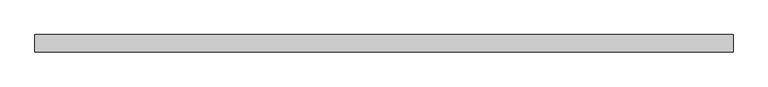
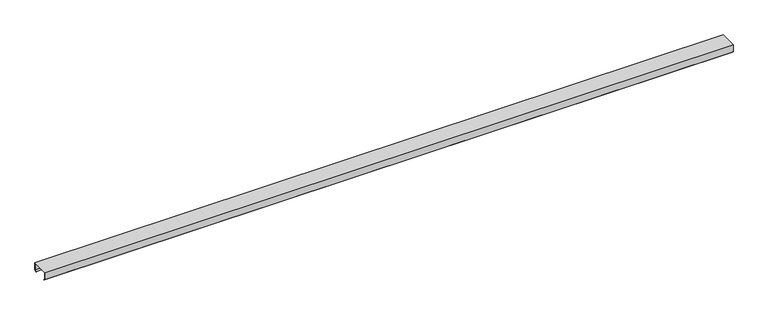
"""IFC4 building model written with IfcOpenShell, lengths in millimetres: proxy geometry, Generic Models 7:Generic Models 1:1:Generic Models 1:1 : Generic Models 7:Generic Models 1:337419:38 : Generic Models 7:Generic Models 1:1:Generic Models 1:1 : Generic Models 7:Generic Models 1:337419:306201."""

from ifc_helpers import new_model, si_unit, frame, origin, place, context, project, spatial, polyline, outline, extrude, source, transform, mapped, element, save


def generic_models_92c28086(model_context):
    return source(origin(), model_context, "Body", "SweptSolid", [
        extrude(outline(polyline([(-578797.4913841, 4985.940625), (-578797.4913841, 4897.040625), (-578812.0845307, 4884.7955211), (-578813.870275, 4886.9236883), (-578800.2695091, 4898.336086), (-578800.2695091, 4983.1625), (-578997.9132591, 4983.1625), (-578997.9132591, 4898.336086), (-578984.3124931, 4886.9236883), (-578986.0982374, 4884.7955211), (-579000.6913841, 4897.040625), (-579000.6913841, 4985.940625), (-578797.4913841, 4985.940625)])), frame((795954.8382438, 0.0, 0.0), z_axis=(1.0, 0.0, 0.0), x_axis=(0.0, 1.0, 0.0)), (0.0, 0.0, 1.0), 8197.85),
    ])


if __name__ == "__main__":
    model = new_model("IFC4")
    model_context = context("Model", 3, world=origin())
    ifc_project = project(units=[si_unit("LENGTHUNIT", "METRE", prefix="MILLI")], contexts=[model_context])
    site = spatial("IfcSite", under=ifc_project)
    building = spatial("IfcBuilding", under=site)
    placement = place(None, origin())
    generic_models_shape = generic_models_92c28086(model_context)
    element("IfcBuildingElementProxy", 1, Name="Generic Models 7:Generic Models 1:1:Generic Models 1:1 : Generic Models 7:Generic Models 1:337419:38 : Generic Models 7:Generic Models 1:1:Generic Models 1:1 : Generic Models 7:Generic Models 1:337419:306201", ObjectType="Generic Models 7:Generic Models 1:1:Generic Models 1:1 : Generic Models 7:Generic Models 1:337419:38 : Generic Models 7:Generic Models 1:1:Generic Models 1:1 : Generic Models 7:Generic Models 1:337419:306201", at=placement, inside=building, context=model_context, shape_type="MappedRepresentation", body=[
        mapped(generic_models_shape, transform((0.0, 0.0, 0.0), x_axis=(1.0, 0.0, 0.0), y_axis=(0.0, 1.0, 0.0), z_axis=(0.0, 0.0, 1.0))),
    ])
    save(model, "model.ifc")

# Revit data of these elements
# Type "Generic Models 7:Generic Models 1:1:Generic Models 1:1 : Generic Models 7:Generic Models 1:337419:38 : Generic Models 7:Generic Models 1:1:Generic Models 1:1 : Generic Models 7:Generic Models 1:337419:306201"
#   NameOverride = "Generic Models 7:Generic Models 1:1:Generic Models 1:1 : Generic Models 7:Generic Models 1:337419:306201"
#   ObjectTypeOverride = "Generic Models 1:1 : Generic Models 7:Generic Models 1:337419"
#   Reference = "Generic Models 1"
#   Tag = "306201"
# Element 1 (IfcBuildingElementProxy, "Generic Models 7:Generic Models 1:1:Generic Models 1:1 : Generic Models 7:Generic Models 1:337419:38 : Generic Models 7:Generic Models 1:1:Generic Models 1:1 : Generic Models 7:Generic Models 1:337419:306201")
#   Materials on its faces: "'ZEE' SECTION (8.0x3.5Z - SEE STRUCT. DWGS)"
# Materials
#   "'ZEE' SECTION (8.0x3.5Z - SEE STRUCT. DWGS)": class "Unassigned", colour RGB 210 209 208, transparency 0, Keynote = "M05121300.02", Cost = 0
